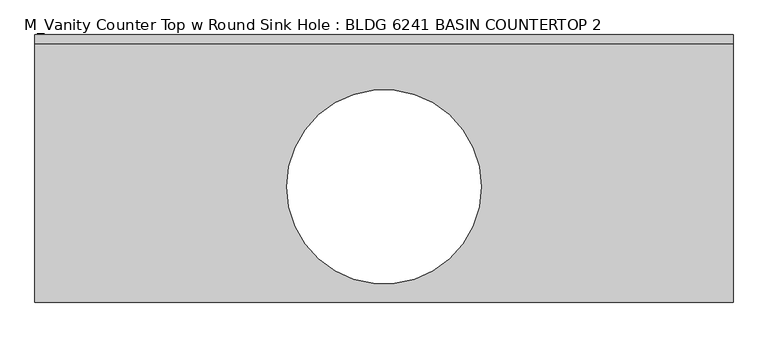
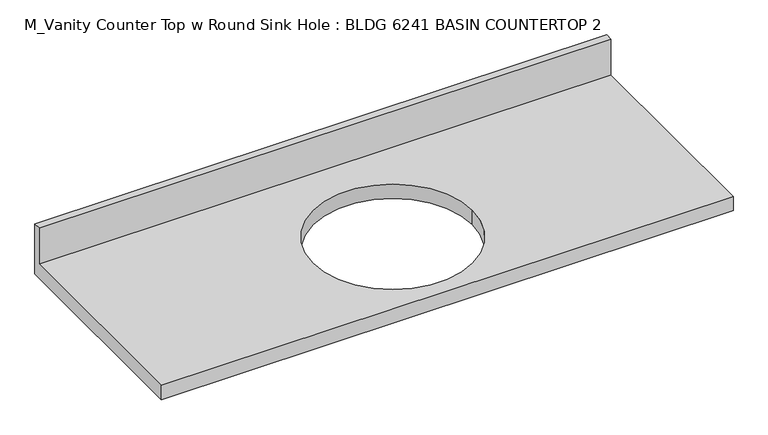
"""IFC4 building model written with IfcOpenShell, lengths in millimetres: furniture geometry, M_Vanity Counter Top w Round Sink Hole : BLDG 6241 BASIN COUNTERTOP 2."""

from ifc_helpers import new_model, si_unit, frame, origin, place, context, project, spatial, polyline, circle_curve, source, transform, mapped, element, save
from ifc_brep_helpers import plane_surface, revolved_surface, advanced_brep


def m_vanity_counter_top_w_round_sink_hole_bldg_6241_basin_d2d8f1b1(model_context):
    return source(origin(), model_context, "Body", "AdvancedBrep", [
        advanced_brep(
        [(-1327.4622951, 0.0, 101.6), (-1327.4622951, -19.05, 101.6), (196.5377049, -19.05, 101.6), (196.5377049, 0.0, 101.6), (-1327.4622951, 0.0, -40.0), (-1327.4622951, -584.2, -40.0), (-1327.4622951, -584.2, 0.0), (-1327.4622951, -19.05, 0.0), (196.5377049, -19.05, 0.0), (196.5377049, -584.2, 0.0), (196.5377049, -584.2, -40.0), (196.5377049, 0.0, -40.0), (-353.1471604, -332.3848653, 0.0), (-777.7774298, -332.3848653, 0.0), (-777.7774298, -332.3848653, -40.0), (-353.1471604, -332.3848653, -40.0)],
        [
            (0, 1),
            (1, 2),
            (2, 3),
            (3, 0),
            (0, 4),
            (4, 5),
            (5, 6),
            (6, 7),
            (7, 1),
            (7, 8),
            (8, 2),
            (8, 9),
            (9, 10),
            (10, 11),
            (11, 3),
            (11, 4),
            (6, 9),
            (12, 13, circle_curve(frame((-565.4622951, -332.3848653, 0.0), z_axis=(0.0, 0.0, -1.0), x_axis=(1.0, 0.0, 0.0)), 212.3151347)),
            (13, 12, circle_curve(frame((-565.4622951, -332.3848653, 0.0), z_axis=(0.0, 0.0, -1.0), x_axis=(1.0, 0.0, 0.0)), 212.3151347)),
            (10, 5),
            (14, 15, circle_curve(frame((-565.4622951, -332.3848653, -40.0), z_axis=(0.0, 0.0, 1.0), x_axis=(1.0, 0.0, 0.0)), 212.3151347)),
            (15, 14, circle_curve(frame((-565.4622951, -332.3848653, -40.0), z_axis=(0.0, 0.0, 1.0), x_axis=(1.0, 0.0, 0.0)), 212.3151347)),
            (12, 15),
            (14, 13),
        ],
        [
            plane_surface(frame((-1327.4622951, 0.0, 101.6), z_axis=(0.0, 0.0, 1.0), x_axis=(0.0, -1.0, 0.0))),
            plane_surface(frame((-1327.4622951, 0.0, 101.6), z_axis=(-1.0, 0.0, 0.0), x_axis=(0.0, 0.0, -1.0))),
            plane_surface(frame((-1327.4622951, -19.05, 101.6), z_axis=(0.0, -1.0, 0.0), x_axis=(0.0, 0.0, -1.0))),
            plane_surface(frame((196.5377049, -19.05, 101.6), z_axis=(1.0, 0.0, 0.0), x_axis=(0.0, 0.0, -1.0))),
            plane_surface(frame((196.5377049, 0.0, 101.6), z_axis=(0.0, 1.0, 0.0), x_axis=(0.0, 0.0, -1.0))),
            plane_surface(frame((-1327.4622951, 0.0, 0.0), z_axis=(0.0, 0.0, 1.0), x_axis=(-1.0, 0.0, 0.0))),
            plane_surface(frame((-1327.4622951, 0.0, -40.0), z_axis=(0.0, 0.0, -1.0), x_axis=(1.0, 0.0, 0.0))),
            plane_surface(frame((-1327.4622951, -584.2, 0.0), z_axis=(0.0, -1.0, 0.0), x_axis=(0.0, 0.0, -1.0))),
            revolved_surface(polyline([(-353.1471604, -332.3848653, 0.0), (-353.1471604, -332.3848653, -40.0)]), (-565.4622951, -332.3848653, -40.0), (0.0, 0.0, 1.0)),
        ],
        [
            (0, [[1, 2, 3, 4]]),
            (1, [[-1, 5, 6, 7, 8, 9]]),
            (2, [[-2, -9, 10, 11]]),
            (3, [[-3, -11, 12, 13, 14, 15]]),
            (4, [[-4, -15, 16, -5]]),
            (5, [[17, -12, -10, -8], [18, 19]]),
            (6, [[-14, 20, -6, -16], [21, 22]]),
            (7, [[-17, -7, -20, -13]]),
            (8, [[23, -21, 24, -18]]),
            (8, [[-23, -19, -24, -22]]),
        ],
    ),
    ])


if __name__ == "__main__":
    model = new_model("IFC4")
    model_context = context("Model", 3, world=origin())
    ifc_project = project(units=[si_unit("LENGTHUNIT", "METRE", prefix="MILLI")], contexts=[model_context])
    site = spatial("IfcSite", under=ifc_project)
    building = spatial("IfcBuilding", under=site)
    placement = place(None, origin())
    m_vanity_counter_top_w_round_sink_hole_bldg_6241_basin_shape = m_vanity_counter_top_w_round_sink_hole_bldg_6241_basin_d2d8f1b1(model_context)
    element("IfcFurniture", 1, ObjectType="M_Vanity Counter Top w Round Sink Hole : BLDG 6241 BASIN COUNTERTOP 2", at=placement, inside=building, context=model_context, shape_type="MappedRepresentation", body=[
        mapped(m_vanity_counter_top_w_round_sink_hole_bldg_6241_basin_shape, transform((0.0, 0.0, 0.0), x_axis=(1.0, 0.0, 0.0), y_axis=(0.0, 1.0, 0.0), z_axis=(0.0, 0.0, 1.0))),
    ])
    save(model, "model.ifc")

# Revit data of these elements
# Type "M_Vanity Counter Top w Round Sink Hole : BLDG 6241 BASIN COUNTERTOP 2"
#   Width = 2' - 6"
#   Default Elevation = 2' - 6"
#   Counter Thickness = 0' - 1.5748"
#   Depth = 1' - 11"
#   Length [instance default] = 3' - 11.24409"
#   Sink Location [instance default] = 1' - 11.62205"
#   Sink Location To Wall [instance default] = 0' - 3.93701"
#   Sink Opening Width [instance default] = 1' - 5.00787"
#   Counter Top Material = none
#   Height = 0
# Element 1 (IfcFurniture, "M_Vanity Counter Top w Round Sink Hole : BLDG 6241 BASIN COUNTERTOP 2")
#   Length = 5' - 0"
#   Sink Location = 2' - 6"
#   Sink Location To Wall = 0' - 5.22715"
#   Sink Opening Width = 1' - 3.71773"
#   Materials on its faces: "Counter Top"
# Materials
#   "Counter Top": class "Wood", colour RGB 226 177 128, transparency 0
